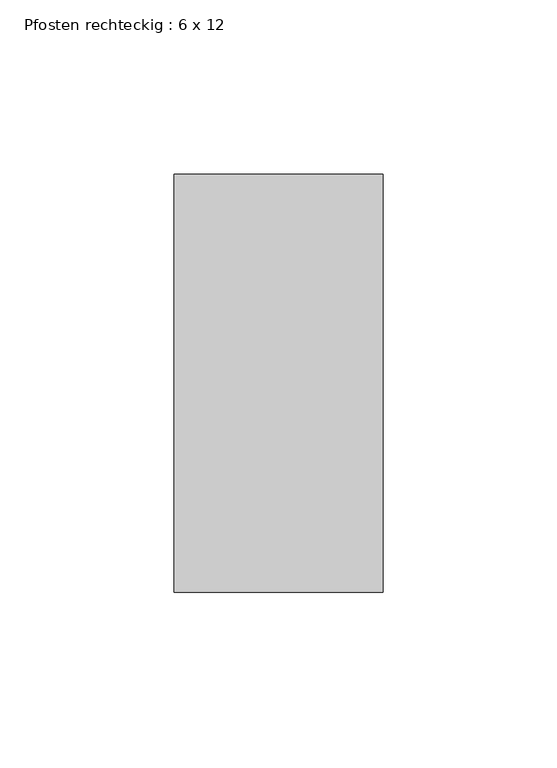
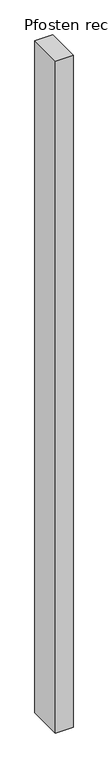
"""IFC4 building model written with IfcOpenShell, lengths in millimetres: member geometry, Pfosten rechteckig : 6 x 12."""

import ifcopenshell
import ifcopenshell.guid

model = None  # the IFC model being written
_history = None  # IfcOwnerHistory: only IFC2X3 demands one
_inside = {}  # id of a spatial element -> (the spatial element, [elements in it])
_under = {}  # id of a project, library or spatial element -> (it, [spatial elements below it])
_declared = {}  # id of a project -> (the project, [libraries it declares])
_typed = {}  # id of a type object -> (the type object, [elements of that type])
_made_of = {}  # id of a material, layer set ... -> (it, [elements and type objects made of it])


def new_model(schema):
    """Start an empty IFC model of exactly this schema.

    Asked for "IFC4X3", IfcOpenShell would pick the latest addendum, in which some entities
    have other attributes; the version numbers below select the first issue.
    IFC2X3 requires an IfcOwnerHistory on every rooted entity: one is made here for all.
    """
    global model, _history
    if schema == "IFC4X3":
        model = ifcopenshell.file(schema_version=(4, 3, 0, 0))
    else:
        model = ifcopenshell.file(schema=schema)
    _inside.clear()
    _under.clear()
    _declared.clear()
    _typed.clear()
    _made_of.clear()
    _history = None
    if model.schema == "IFC2X3":
        org = make("IfcOrganization", Name="unknown")
        user = make(
            "IfcPersonAndOrganization",
            ThePerson=make("IfcPerson", FamilyName="unknown"),
            TheOrganization=org,
        )
        app = make(
            "IfcApplication",
            ApplicationDeveloper=org,
            Version="unknown",
            ApplicationFullName="unknown",
            ApplicationIdentifier="unknown",
        )
        _history = make(
            "IfcOwnerHistory",
            OwningUser=user,
            OwningApplication=app,
            ChangeAction="ADDED",
            CreationDate=0,
        )
    return model


def make(cls, **values):
    """One entity of the class cls with the attributes given. An attribute that is None is left unset."""
    return model.create_entity(
        cls, **{name: value for name, value in values.items() if value is not None}
    )


def rooted(cls, **values):
    """An entity with a GlobalId (a new one), such as an element, a storey or a relation."""
    return make(cls, GlobalId=ifcopenshell.guid.new(), OwnerHistory=_history, **values)


def si_unit(unit_type, name, prefix=None):
    """IfcSIUnit, for example si_unit("LENGTHUNIT", "METRE", prefix="MILLI")."""
    return make("IfcSIUnit", UnitType=unit_type, Prefix=prefix, Name=name)


def assignment(units):
    """IfcUnitAssignment: the units of a project."""
    return None if units is None else make("IfcUnitAssignment", Units=units)


def point(xyz):
    """IfcCartesianPoint."""
    return None if xyz is None else make("IfcCartesianPoint", Coordinates=xyz)


def direction(xyz):
    """IfcDirection."""
    return None if xyz is None else make("IfcDirection", DirectionRatios=xyz)


def frame(location, z_axis=None, x_axis=None):
    """IfcAxis2Placement3D, a coordinate frame: its origin and axes. An axis left out is left unset."""
    return make(
        "IfcAxis2Placement3D",
        Location=point(location),
        Axis=direction(z_axis),
        RefDirection=direction(x_axis),
    )


def origin():
    """The frame at (0, 0, 0) with its axes left unset."""
    return frame((0.0, 0.0, 0.0))


def place(relative_to, where):
    """IfcLocalPlacement: puts the frame where relative to a parent placement (None: the world)."""
    return make(
        "IfcLocalPlacement", PlacementRelTo=relative_to, RelativePlacement=where
    )


def context(
    kind, dimensions, precision=None, world=None, true_north=None, identifier=None
):
    """IfcGeometricRepresentationContext, for example the 3D "Model" context."""
    return make(
        "IfcGeometricRepresentationContext",
        ContextIdentifier=identifier,
        ContextType=kind,
        CoordinateSpaceDimension=dimensions,
        Precision=precision,
        WorldCoordinateSystem=world,
        TrueNorth=true_north,
    )


def project(units=None, contexts=None):
    """IfcProject with its units and contexts."""
    return rooted(
        "IfcProject",
        Name="project",
        RepresentationContexts=contexts,
        UnitsInContext=assignment(units),
    )


def spatial(cls, under=None, at=None, **own):
    """A site, building, storey or space (cls), placed at a placement, below another one or the project."""
    s = rooted(cls, ObjectPlacement=at, **own)
    if under is not None:
        _under.setdefault(under.id(), (under, []))[1].append(s)
    return s


def polyline(points):
    """IfcPolyline through the points."""
    return make("IfcPolyline", Points=[point(p) for p in points])


def outline(outer, holes=None, kind="AREA"):
    """IfcArbitraryClosedProfileDef: a profile drawn as a closed curve; with holes, ...WithVoids."""
    if holes is None:
        return make("IfcArbitraryClosedProfileDef", ProfileType=kind, OuterCurve=outer)
    return make(
        "IfcArbitraryProfileDefWithVoids",
        ProfileType=kind,
        OuterCurve=outer,
        InnerCurves=holes,
    )


def extrude(swept, where, along, depth):
    """IfcExtrudedAreaSolid: the profile swept, set in the frame where, extruded along a direction by depth."""
    return make(
        "IfcExtrudedAreaSolid",
        SweptArea=swept,
        Position=where,
        ExtrudedDirection=direction(along),
        Depth=depth,
    )


def shape(context_of_items, identifier, shape_type, items):
    """IfcShapeRepresentation: the items that make up one representation, for example the "Body"."""
    return make(
        "IfcShapeRepresentation",
        ContextOfItems=context_of_items,
        RepresentationIdentifier=identifier,
        RepresentationType=shape_type,
        Items=items,
    )


def source(mapping_origin, context_of_items, identifier, shape_type, items):
    """IfcRepresentationMap: a shape defined once, which mapped items show again and again."""
    return make(
        "IfcRepresentationMap",
        MappingOrigin=mapping_origin,
        MappedRepresentation=shape(context_of_items, identifier, shape_type, items),
    )


def transform(
    local_origin,
    x_axis=None,
    y_axis=None,
    z_axis=None,
    scale=None,
    scale2=None,
    scale3=None,
    uniform=True,
):
    """IfcCartesianTransformationOperator3D, or its non-uniform kind. x_axis, y_axis, z_axis: its Axis1, 2, 3."""
    if uniform:
        return make(
            "IfcCartesianTransformationOperator3D",
            Axis1=direction(x_axis),
            Axis2=direction(y_axis),
            LocalOrigin=point(local_origin),
            Scale=scale,
            Axis3=direction(z_axis),
        )
    return make(
        "IfcCartesianTransformationOperator3DnonUniform",
        Axis1=direction(x_axis),
        Axis2=direction(y_axis),
        LocalOrigin=point(local_origin),
        Scale=scale,
        Axis3=direction(z_axis),
        Scale2=scale2,
        Scale3=scale3,
    )


def mapped(mapping_source, mapping_target):
    """IfcMappedItem: shows the shape of a source again, moved by a transform."""
    return make(
        "IfcMappedItem", MappingSource=mapping_source, MappingTarget=mapping_target
    )


def made_of(thing, what):
    """Note that an element or type object is made of a material, layer set ...; save() writes the relation."""
    if what is not None:
        _made_of.setdefault(what.id(), (what, []))[1].append(thing)
    return thing


def element(
    cls,
    number,
    at=None,
    inside=None,
    cuts=None,
    type_object=None,
    material=None,
    context=None,
    identifier="Body",
    shape_type=None,
    held_by="IfcProductDefinitionShape",
    body=None,
    shapes=None,
    **own,
):
    """One element of the class cls, such as IfcWall. Its Tag is "e" and its number.

    at: its placement. inside: the storey or other place that contains it. cuts: it is an
    opening in that element (IfcRelVoidsElement). A single representation is given by context,
    identifier, shape_type and body (its items); several are given by shapes. held_by: the class
    of the entity that holds the representations. save() writes the other relations.
    """
    e = rooted(cls, Tag="e%d" % number, ObjectPlacement=at, **own)
    if body is not None:
        shapes = [shape(context, identifier, shape_type, body)]
    if shapes is not None:
        e.Representation = make(held_by, Representations=shapes)
    if inside is not None:
        _inside.setdefault(inside.id(), (inside, []))[1].append(e)
    if cuts is not None:
        rooted(
            "IfcRelVoidsElement", RelatingBuildingElement=cuts, RelatedOpeningElement=e
        )
    if type_object is not None:
        _typed.setdefault(type_object.id(), (type_object, []))[1].append(e)
    return made_of(e, material)


def aggregate(whole, parts):
    """IfcRelAggregates: a whole, such as a stair, and the parts it consists of."""
    return rooted("IfcRelAggregates", RelatingObject=whole, RelatedObjects=parts)


def save(model, path):
    """Write the relations noted so far, then the file.

    IfcRelAggregates (storeys below a building ...), IfcRelContainedInSpatialStructure (elements
    in a storey), IfcRelDefinesByType, IfcRelAssociatesMaterial and IfcRelDeclares: one each for
    every whole, place, type object, material and project.
    """
    for whole, parts in _under.values():
        aggregate(whole, parts)
    for where, things in _inside.values():
        rooted(
            "IfcRelContainedInSpatialStructure",
            RelatedElements=things,
            RelatingStructure=where,
        )
    for kind, things in _typed.values():
        rooted("IfcRelDefinesByType", RelatedObjects=things, RelatingType=kind)
    for what, things in _made_of.values():
        rooted("IfcRelAssociatesMaterial", RelatedObjects=things, RelatingMaterial=what)
    for by, libraries in _declared.values():
        rooted("IfcRelDeclares", RelatingContext=by, RelatedDefinitions=libraries)
    model.write(path)


def pfosten_rechteckig_6_x_12_68950c07(model_context):
    return source(origin(), model_context, "Body", "SweptSolid", [
        extrude(outline(polyline([(0.0, 60.0), (0.0, -60.0), (-60.0, -60.0), (-60.0, 60.0), (0.0, 60.0)])), frame((0.0, 0.0, -2410.0000003), z_axis=(0.0, 0.0, 1.0), x_axis=(1.0, 0.0, 0.0)), (0.0, 0.0, 1.0), 2410.0000003),
    ])


if __name__ == "__main__":
    model = new_model("IFC4")
    model_context = context("Model", 3, world=origin())
    ifc_project = project(units=[si_unit("LENGTHUNIT", "METRE", prefix="MILLI")], contexts=[model_context])
    site = spatial("IfcSite", under=ifc_project)
    building = spatial("IfcBuilding", under=site)
    placement = place(None, origin())
    pfosten_rechteckig_6_x_12_shape = pfosten_rechteckig_6_x_12_68950c07(model_context)
    element("IfcMember", 1, ObjectType="Pfosten rechteckig : 6 x 12", at=placement, inside=building, context=model_context, shape_type="MappedRepresentation", body=[
        mapped(pfosten_rechteckig_6_x_12_shape, transform((0.0, 0.0, 0.0), x_axis=(1.0, 0.0, 0.0), y_axis=(0.0, 1.0, 0.0), z_axis=(0.0, 0.0, 1.0))),
    ])
    save(model, "model.ifc")

# Revit data of these elements
# Type "Pfosten rechteckig : 6 x 12"
#   built-in parameter 1007304 = 0.393701 (stored number, unit not read)
#   built-in parameter 1007301 = 0.0984252 (stored number, unit not read)
#   built-in parameter 1007300 = 0.0984252 (stored number, unit not read)
# Element 1 (IfcMember, "Pfosten rechteckig : 6 x 12")
#   Materials on its faces: "Metall - verzinkt"
# Materials
#   "Metall - verzinkt": class "Allgemeines", colour RGB 200 200 200, transparency 0, Cost = 0
